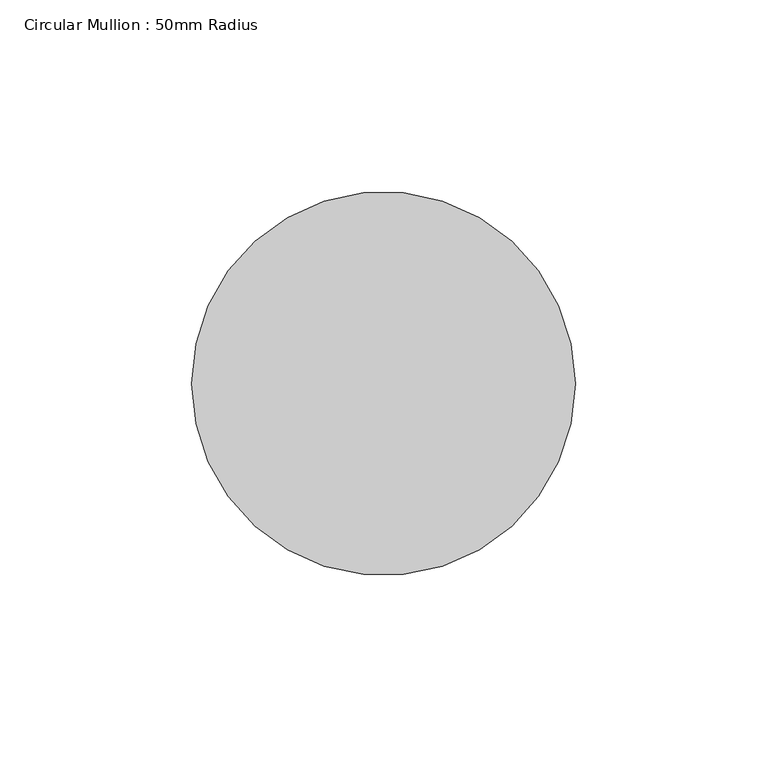
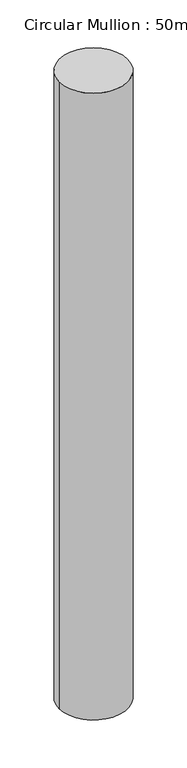
"""IFC4 building model written with IfcOpenShell, lengths in millimetres: member geometry, Circular Mullion : 50mm Radius."""

from ifc_helpers import new_model, si_unit, point, frame, origin, origin_2d, place, context, project, spatial, circle_curve, trimmed, segment, composite_curve, outline, extrude, source, transform, mapped, element, save


def circular_mullion_50mm_radius_b6edca98(model_context):
    return source(origin(), model_context, "Body", "SweptSolid", [
        extrude(outline(composite_curve([segment(trimmed(circle_curve(origin_2d(), 50.0), [point((50.0, 0.0))], [point((-50.0, 0.0))], False, "CARTESIAN"), True, "CONTINUOUS"), segment(trimmed(circle_curve(origin_2d(), 50.0), [point((-50.0, 0.0))], [point((50.0, 0.0))], False, "CARTESIAN"), True, "CONTINUOUS")], self_intersect=False)), frame((0.0, 0.0, -966.2384977), z_axis=(0.0, 0.0, 1.0), x_axis=(1.0, 0.0, 0.0)), (0.0, 0.0, 1.0), 966.2384977),
    ])


if __name__ == "__main__":
    model = new_model("IFC4")
    model_context = context("Model", 3, world=origin())
    ifc_project = project(units=[si_unit("LENGTHUNIT", "METRE", prefix="MILLI")], contexts=[model_context])
    site = spatial("IfcSite", under=ifc_project)
    building = spatial("IfcBuilding", under=site)
    placement = place(None, origin())
    circular_mullion_50mm_radius_shape = circular_mullion_50mm_radius_b6edca98(model_context)
    element("IfcMember", 1, ObjectType="Circular Mullion : 50mm Radius", at=placement, inside=building, context=model_context, shape_type="MappedRepresentation", body=[
        mapped(circular_mullion_50mm_radius_shape, transform((0.0, 0.0, 0.0), x_axis=(1.0, 0.0, 0.0), y_axis=(0.0, 1.0, 0.0), z_axis=(0.0, 0.0, 1.0))),
    ])
    save(model, "model.ifc")

# Revit data of these elements
# Type "Circular Mullion : 50mm Radius"
#   built-in parameter 1007350 = 0.164042 (stored number, unit not read)
# Element 1 (IfcMember, "Circular Mullion : 50mm Radius")
#   Materials on its faces: "Aluminium"
# Materials
#   "Aluminium": class "Metal", colour RGB 247 247 247, transparency 0, Description = "Aluminium 6061", Cost = 0
